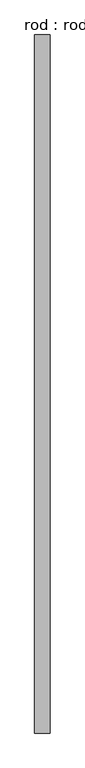
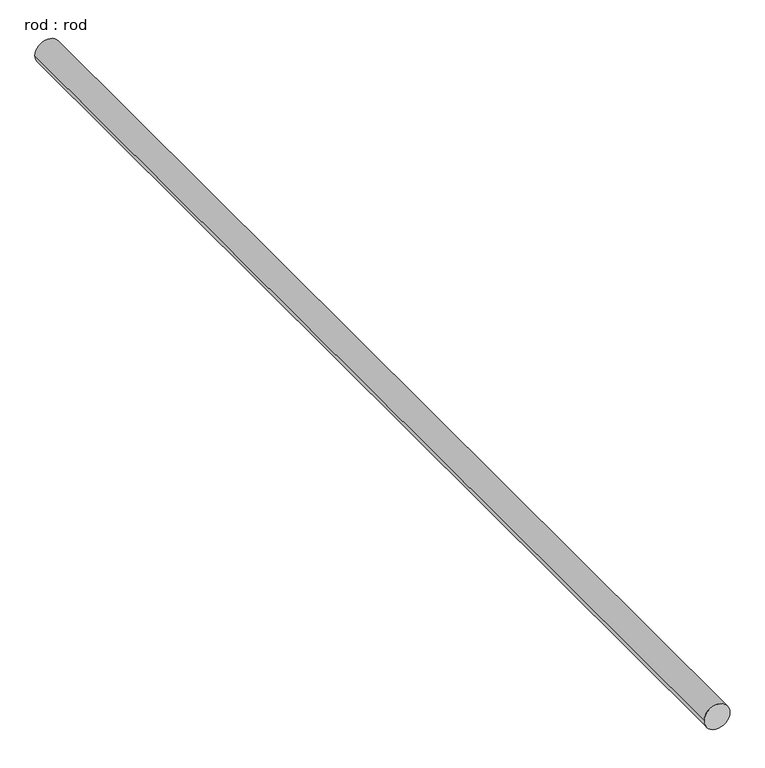
"""IFC4 building model written with IfcOpenShell, lengths in millimetres: proxy geometry, rod : rod."""

from ifc_helpers import new_model, si_unit, point, frame, frame_2d, origin, place, context, project, spatial, circle_curve, trimmed, segment, composite_curve, outline, extrude, source, transform, mapped, element, save


def rod_rod_6da7ea00(model_context):
    return source(origin(), model_context, "Body", "SweptSolid", [
        extrude(outline(composite_curve([segment(trimmed(circle_curve(frame_2d((0.0108462, 0.0)), 200.0), [point((0.0108462, 200.0))], [point((0.0108462, -200.0))], False, "CARTESIAN"), True, "CONTINUOUS"), segment(trimmed(circle_curve(frame_2d((0.0108462, 0.0)), 200.0), [point((0.0108462, -200.0))], [point((0.0108462, 200.0))], False, "CARTESIAN"), True, "CONTINUOUS")], self_intersect=False)), frame((0.0, -4901.5086515, 0.0), z_axis=(0.0, 1.0, 0.0), x_axis=(0.0, 0.0, 1.0)), (0.0, 0.0, 1.0), 17988.4745337),
    ])


if __name__ == "__main__":
    model = new_model("IFC4")
    model_context = context("Model", 3, world=origin())
    ifc_project = project(units=[si_unit("LENGTHUNIT", "METRE", prefix="MILLI")], contexts=[model_context])
    site = spatial("IfcSite", under=ifc_project)
    building = spatial("IfcBuilding", under=site)
    placement = place(None, origin())
    rod_rod_shape = rod_rod_6da7ea00(model_context)
    element("IfcBuildingElementProxy", 1, Name="rod : rod", ObjectType="rod : rod", at=placement, inside=building, context=model_context, shape_type="MappedRepresentation", body=[
        mapped(rod_rod_shape, transform((0.0, 0.0, 0.0), x_axis=(1.0, 0.0, 0.0), y_axis=(0.0, 1.0, 0.0), z_axis=(0.0, 0.0, 1.0))),
    ])
    save(model, "model.ifc")

# Revit data of these elements
# Type "rod : rod"
#   Default Elevation = 0
